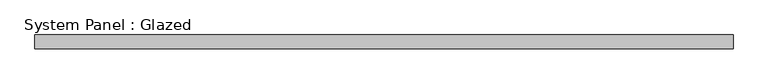
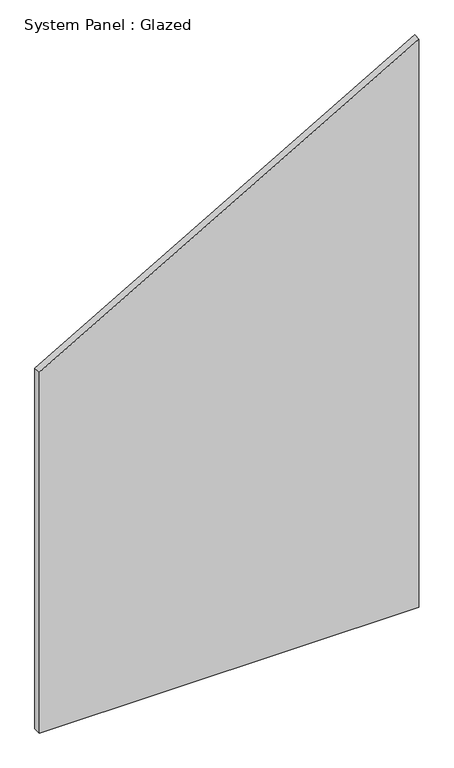
"""IFC4 building model written with IfcOpenShell, lengths in millimetres: plate geometry, System Panel : Glazed."""

from ifc_helpers import new_model, si_unit, frame, origin, place, context, project, spatial, polyline, outline, extrude, source, transform, mapped, element, save


def system_panel_glazed_d3b5986c(model_context):
    return source(origin(), model_context, "Body", "SweptSolid", [
        extrude(outline(polyline([(0.0, -639.2857142), (0.0, 639.2857142), (2022.5740063, 639.2857142), (1284.3904479, -639.2857142), (0.0, -639.2857142)])), frame((0.0, 24.5, 0.0), z_axis=(0.0, 1.0, 0.0), x_axis=(0.0, 0.0, 1.0)), (0.0, 0.0, 1.0), 25.0),
    ])


if __name__ == "__main__":
    model = new_model("IFC4")
    model_context = context("Model", 3, world=origin())
    ifc_project = project(units=[si_unit("LENGTHUNIT", "METRE", prefix="MILLI")], contexts=[model_context])
    site = spatial("IfcSite", under=ifc_project)
    building = spatial("IfcBuilding", under=site)
    placement = place(None, origin())
    system_panel_glazed_shape = system_panel_glazed_d3b5986c(model_context)
    element("IfcPlate", 1, ObjectType="System Panel : Glazed", at=placement, inside=building, context=model_context, shape_type="MappedRepresentation", body=[
        mapped(system_panel_glazed_shape, transform((0.0, 0.0, 0.0), x_axis=(1.0, 0.0, 0.0), y_axis=(0.0, 1.0, 0.0), z_axis=(0.0, 0.0, 1.0))),
    ])
    save(model, "model.ifc")

# Revit data of these elements
# Type "System Panel : Glazed"
#   Construction Type Id = "GSP4R"
#   Analytic Construction = "1/8 in Pilkington single glazing"
#   Visual Light Transmittance = 0.9
#   Solar Heat Gain Coefficient = 0.86
#   Heat Transfer Coefficient (U) = 6.7069 W/(m²·K)
#   Define Thermal Properties by = 1
# Element 1 (IfcPlate, "System Panel : Glazed")
#   Materials on its faces: "Glass"
# Materials
#   "Glass": class "Glass", colour RGB 0 128 192, transparency 0.75, Description = "Soda Lime Glass", Cost = 0
